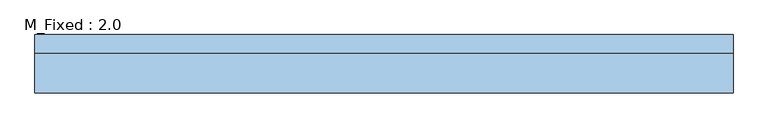
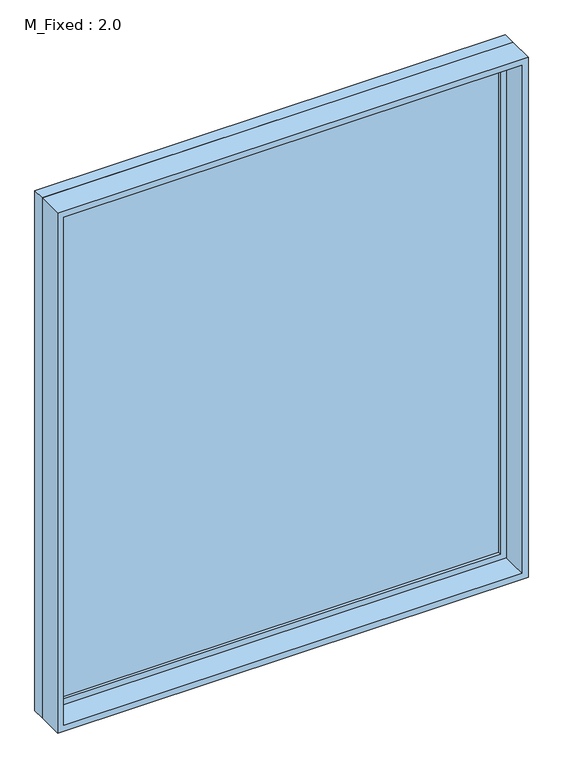
"""IFC4 building model written with IfcOpenShell, lengths in millimetres: window geometry, M_Fixed : 2.0."""

from ifc_helpers import new_model, si_unit, frame, origin, place, context, project, spatial, polyline, outline, extrude, source, transform, mapped, element, save


def m_fixed_2_0_adb39516(model_context):
    return source(origin(), model_context, "Body", "SweptSolid", [
        extrude(outline(polyline([(-1137.0, 78.0), (1137.0, 78.0), (1137.0, 66.0), (-1137.0, 66.0), (-1137.0, 78.0)])), frame((0.0, 0.0, 978.0), z_axis=(0.0, 0.0, 1.0), x_axis=(1.0, 0.0, 0.0)), (0.0, 0.0, 1.0), 2674.0),
        extrude(outline(polyline([(3696.0, -1181.0), (934.0, -1181.0), (934.0, 1181.0), (3696.0, 1181.0), (3696.0, -1181.0)]), holes=[polyline([(3652.0, -1137.0), (3652.0, 1137.0), (978.0, 1137.0), (978.0, -1137.0), (3652.0, -1137.0)])]), frame((0.0, 50.0, 0.0), z_axis=(0.0, 1.0, 0.0), x_axis=(0.0, 0.0, 1.0)), (0.0, 0.0, 1.0), 44.0),
        extrude(outline(polyline([(3715.0, -1200.0), (915.0, -1200.0), (915.0, 1200.0), (3715.0, 1200.0), (3715.0, -1200.0)]), holes=[polyline([(3696.0, -1181.0), (3696.0, 1181.0), (934.0, 1181.0), (934.0, -1181.0), (3696.0, -1181.0)])]), frame((0.0, 50.0, 0.0), z_axis=(0.0, 1.0, 0.0), x_axis=(0.0, 0.0, 1.0)), (0.0, 0.0, 1.0), 63.0),
        extrude(outline(polyline([(3715.0, -1200.0), (915.0, -1200.0), (915.0, 1200.0), (3715.0, 1200.0), (3715.0, -1200.0)]), holes=[polyline([(3683.0, -1168.0), (3683.0, 1168.0), (947.0, 1168.0), (947.0, -1168.0), (3683.0, -1168.0)])]), frame((0.0, -87.0, 0.0), z_axis=(0.0, 1.0, 0.0), x_axis=(0.0, 0.0, 1.0)), (0.0, 0.0, 1.0), 137.0),
    ])


if __name__ == "__main__":
    model = new_model("IFC4")
    model_context = context("Model", 3, world=origin())
    ifc_project = project(units=[si_unit("LENGTHUNIT", "METRE", prefix="MILLI")], contexts=[model_context])
    site = spatial("IfcSite", under=ifc_project)
    building = spatial("IfcBuilding", under=site)
    placement = place(None, origin())
    m_fixed_2_0_shape = m_fixed_2_0_adb39516(model_context)
    element("IfcWindow", 1, ObjectType="M_Fixed : 2.0", at=placement, inside=building, context=model_context, shape_type="MappedRepresentation", body=[
        mapped(m_fixed_2_0_shape, transform((0.0, 0.0, 0.0), x_axis=(1.0, 0.0, 0.0), y_axis=(0.0, 1.0, 0.0), z_axis=(0.0, 0.0, 1.0))),
    ])
    save(model, "model.ifc")

# Revit data of these elements
# Type "M_Fixed : 2.0"
#   Type Mark = "19"
#   Height = 2.8 m
#   Default Sill Height = 0.915 m
#   Width = 2.4 m
#   Window Inset = 0.019 m
#   Frame Exterior Material = Glass
#   Frame Interior Material = Sash
#   Glass Pane Material = Glass
#   Sash = Sash
#   Wall Closure = (empty or 0)
# Element 1 (IfcWindow, "M_Fixed : 2.0")
#   Materials on its faces: "Sash", "Glass"
# Materials
#   "Glass": class "Glass", colour RGB 218 227 224, transparency 0.85, Description = "Soda Lime Glass", Cost = 0
#   "Sash": class "Wood", colour RGB 136 99 55, transparency 0, Cost = 0
